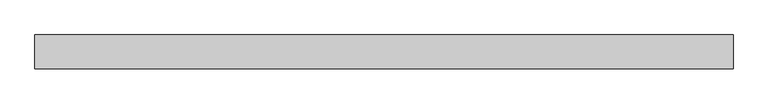
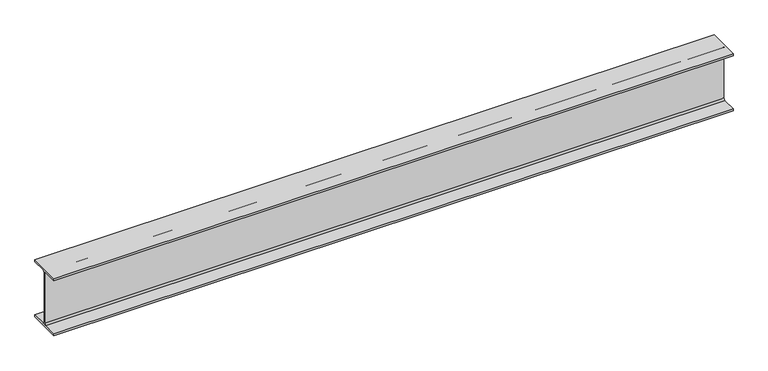
"""IFC4 building model written with IfcOpenShell, lengths in millimetres: beam geometry, Old_Steel Beam_H-KSD3502 : H_SB_ASB_H-200×200x8x12."""

import ifcopenshell
import ifcopenshell.guid

model = None  # the IFC model being written
_history = None  # IfcOwnerHistory: only IFC2X3 demands one
_inside = {}  # id of a spatial element -> (the spatial element, [elements in it])
_under = {}  # id of a project, library or spatial element -> (it, [spatial elements below it])
_declared = {}  # id of a project -> (the project, [libraries it declares])
_typed = {}  # id of a type object -> (the type object, [elements of that type])
_made_of = {}  # id of a material, layer set ... -> (it, [elements and type objects made of it])


def new_model(schema):
    """Start an empty IFC model of exactly this schema.

    Asked for "IFC4X3", IfcOpenShell would pick the latest addendum, in which some entities
    have other attributes; the version numbers below select the first issue.
    IFC2X3 requires an IfcOwnerHistory on every rooted entity: one is made here for all.
    """
    global model, _history
    if schema == "IFC4X3":
        model = ifcopenshell.file(schema_version=(4, 3, 0, 0))
    else:
        model = ifcopenshell.file(schema=schema)
    _inside.clear()
    _under.clear()
    _declared.clear()
    _typed.clear()
    _made_of.clear()
    _history = None
    if model.schema == "IFC2X3":
        org = make("IfcOrganization", Name="unknown")
        user = make(
            "IfcPersonAndOrganization",
            ThePerson=make("IfcPerson", FamilyName="unknown"),
            TheOrganization=org,
        )
        app = make(
            "IfcApplication",
            ApplicationDeveloper=org,
            Version="unknown",
            ApplicationFullName="unknown",
            ApplicationIdentifier="unknown",
        )
        _history = make(
            "IfcOwnerHistory",
            OwningUser=user,
            OwningApplication=app,
            ChangeAction="ADDED",
            CreationDate=0,
        )
    return model


def make(cls, **values):
    """One entity of the class cls with the attributes given. An attribute that is None is left unset."""
    return model.create_entity(
        cls, **{name: value for name, value in values.items() if value is not None}
    )


def rooted(cls, **values):
    """An entity with a GlobalId (a new one), such as an element, a storey or a relation."""
    return make(cls, GlobalId=ifcopenshell.guid.new(), OwnerHistory=_history, **values)


def si_unit(unit_type, name, prefix=None):
    """IfcSIUnit, for example si_unit("LENGTHUNIT", "METRE", prefix="MILLI")."""
    return make("IfcSIUnit", UnitType=unit_type, Prefix=prefix, Name=name)


def assignment(units):
    """IfcUnitAssignment: the units of a project."""
    return None if units is None else make("IfcUnitAssignment", Units=units)


def point(xyz):
    """IfcCartesianPoint."""
    return None if xyz is None else make("IfcCartesianPoint", Coordinates=xyz)


def direction(xyz):
    """IfcDirection."""
    return None if xyz is None else make("IfcDirection", DirectionRatios=xyz)


def frame(location, z_axis=None, x_axis=None):
    """IfcAxis2Placement3D, a coordinate frame: its origin and axes. An axis left out is left unset."""
    return make(
        "IfcAxis2Placement3D",
        Location=point(location),
        Axis=direction(z_axis),
        RefDirection=direction(x_axis),
    )


def frame_2d(location, x_axis=None):
    """IfcAxis2Placement2D, a coordinate frame in the plane: its origin and x axis."""
    return make(
        "IfcAxis2Placement2D", Location=point(location), RefDirection=direction(x_axis)
    )


def origin():
    """The frame at (0, 0, 0) with its axes left unset."""
    return frame((0.0, 0.0, 0.0))


def place(relative_to, where):
    """IfcLocalPlacement: puts the frame where relative to a parent placement (None: the world)."""
    return make(
        "IfcLocalPlacement", PlacementRelTo=relative_to, RelativePlacement=where
    )


def context(
    kind, dimensions, precision=None, world=None, true_north=None, identifier=None
):
    """IfcGeometricRepresentationContext, for example the 3D "Model" context."""
    return make(
        "IfcGeometricRepresentationContext",
        ContextIdentifier=identifier,
        ContextType=kind,
        CoordinateSpaceDimension=dimensions,
        Precision=precision,
        WorldCoordinateSystem=world,
        TrueNorth=true_north,
    )


def project(units=None, contexts=None):
    """IfcProject with its units and contexts."""
    return rooted(
        "IfcProject",
        Name="project",
        RepresentationContexts=contexts,
        UnitsInContext=assignment(units),
    )


def spatial(cls, under=None, at=None, **own):
    """A site, building, storey or space (cls), placed at a placement, below another one or the project."""
    s = rooted(cls, ObjectPlacement=at, **own)
    if under is not None:
        _under.setdefault(under.id(), (under, []))[1].append(s)
    return s


def polyline(points):
    """IfcPolyline through the points."""
    return make("IfcPolyline", Points=[point(p) for p in points])


def circle_curve(where, radius):
    """IfcCircle in the frame where."""
    return make("IfcCircle", Position=where, Radius=radius)


def trimmed(basis, trim1, trim2, sense, master):
    """IfcTrimmedCurve: the piece of a basis curve between two trims."""
    return make(
        "IfcTrimmedCurve",
        BasisCurve=basis,
        Trim1=trim1,
        Trim2=trim2,
        SenseAgreement=sense,
        MasterRepresentation=master,
    )


def segment(curve, same_sense, transition):
    """IfcCompositeCurveSegment."""
    return make(
        "IfcCompositeCurveSegment",
        Transition=transition,
        SameSense=same_sense,
        ParentCurve=curve,
    )


def composite_curve(segments, self_intersect=None):
    """IfcCompositeCurve: segments joined end to end."""
    return make("IfcCompositeCurve", Segments=segments, SelfIntersect=self_intersect)


def outline(outer, holes=None, kind="AREA"):
    """IfcArbitraryClosedProfileDef: a profile drawn as a closed curve; with holes, ...WithVoids."""
    if holes is None:
        return make("IfcArbitraryClosedProfileDef", ProfileType=kind, OuterCurve=outer)
    return make(
        "IfcArbitraryProfileDefWithVoids",
        ProfileType=kind,
        OuterCurve=outer,
        InnerCurves=holes,
    )


def extrude(swept, where, along, depth):
    """IfcExtrudedAreaSolid: the profile swept, set in the frame where, extruded along a direction by depth."""
    return make(
        "IfcExtrudedAreaSolid",
        SweptArea=swept,
        Position=where,
        ExtrudedDirection=direction(along),
        Depth=depth,
    )


def shape(context_of_items, identifier, shape_type, items):
    """IfcShapeRepresentation: the items that make up one representation, for example the "Body"."""
    return make(
        "IfcShapeRepresentation",
        ContextOfItems=context_of_items,
        RepresentationIdentifier=identifier,
        RepresentationType=shape_type,
        Items=items,
    )


def source(mapping_origin, context_of_items, identifier, shape_type, items):
    """IfcRepresentationMap: a shape defined once, which mapped items show again and again."""
    return make(
        "IfcRepresentationMap",
        MappingOrigin=mapping_origin,
        MappedRepresentation=shape(context_of_items, identifier, shape_type, items),
    )


def transform(
    local_origin,
    x_axis=None,
    y_axis=None,
    z_axis=None,
    scale=None,
    scale2=None,
    scale3=None,
    uniform=True,
):
    """IfcCartesianTransformationOperator3D, or its non-uniform kind. x_axis, y_axis, z_axis: its Axis1, 2, 3."""
    if uniform:
        return make(
            "IfcCartesianTransformationOperator3D",
            Axis1=direction(x_axis),
            Axis2=direction(y_axis),
            LocalOrigin=point(local_origin),
            Scale=scale,
            Axis3=direction(z_axis),
        )
    return make(
        "IfcCartesianTransformationOperator3DnonUniform",
        Axis1=direction(x_axis),
        Axis2=direction(y_axis),
        LocalOrigin=point(local_origin),
        Scale=scale,
        Axis3=direction(z_axis),
        Scale2=scale2,
        Scale3=scale3,
    )


def mapped(mapping_source, mapping_target):
    """IfcMappedItem: shows the shape of a source again, moved by a transform."""
    return make(
        "IfcMappedItem", MappingSource=mapping_source, MappingTarget=mapping_target
    )


def made_of(thing, what):
    """Note that an element or type object is made of a material, layer set ...; save() writes the relation."""
    if what is not None:
        _made_of.setdefault(what.id(), (what, []))[1].append(thing)
    return thing


def element(
    cls,
    number,
    at=None,
    inside=None,
    cuts=None,
    type_object=None,
    material=None,
    context=None,
    identifier="Body",
    shape_type=None,
    held_by="IfcProductDefinitionShape",
    body=None,
    shapes=None,
    **own,
):
    """One element of the class cls, such as IfcWall. Its Tag is "e" and its number.

    at: its placement. inside: the storey or other place that contains it. cuts: it is an
    opening in that element (IfcRelVoidsElement). A single representation is given by context,
    identifier, shape_type and body (its items); several are given by shapes. held_by: the class
    of the entity that holds the representations. save() writes the other relations.
    """
    e = rooted(cls, Tag="e%d" % number, ObjectPlacement=at, **own)
    if body is not None:
        shapes = [shape(context, identifier, shape_type, body)]
    if shapes is not None:
        e.Representation = make(held_by, Representations=shapes)
    if inside is not None:
        _inside.setdefault(inside.id(), (inside, []))[1].append(e)
    if cuts is not None:
        rooted(
            "IfcRelVoidsElement", RelatingBuildingElement=cuts, RelatedOpeningElement=e
        )
    if type_object is not None:
        _typed.setdefault(type_object.id(), (type_object, []))[1].append(e)
    return made_of(e, material)


def aggregate(whole, parts):
    """IfcRelAggregates: a whole, such as a stair, and the parts it consists of."""
    return rooted("IfcRelAggregates", RelatingObject=whole, RelatedObjects=parts)


def save(model, path):
    """Write the relations noted so far, then the file.

    IfcRelAggregates (storeys below a building ...), IfcRelContainedInSpatialStructure (elements
    in a storey), IfcRelDefinesByType, IfcRelAssociatesMaterial and IfcRelDeclares: one each for
    every whole, place, type object, material and project.
    """
    for whole, parts in _under.values():
        aggregate(whole, parts)
    for where, things in _inside.values():
        rooted(
            "IfcRelContainedInSpatialStructure",
            RelatedElements=things,
            RelatingStructure=where,
        )
    for kind, things in _typed.values():
        rooted("IfcRelDefinesByType", RelatedObjects=things, RelatingType=kind)
    for what, things in _made_of.values():
        rooted("IfcRelAssociatesMaterial", RelatedObjects=things, RelatingMaterial=what)
    for by, libraries in _declared.values():
        rooted("IfcRelDeclares", RelatingContext=by, RelatedDefinitions=libraries)
    model.write(path)


def beam_af1dc2e2(model_context):
    return source(origin(), model_context, "Body", "SweptSolid", [
        extrude(outline(composite_curve([segment(polyline([(-82.5, -141.5), (-11.9, -141.5)]), True, "CONTINUOUS"), segment(trimmed(circle_curve(frame_2d((-11.9, -132.6)), 8.9), [point((-11.9, -141.5))], [point((-3.0, -132.6))], True, "CARTESIAN"), True, "CONTINUOUS"), segment(polyline([(-3.0, -132.6), (-3.0, 132.6)]), True, "CONTINUOUS"), segment(trimmed(circle_curve(frame_2d((-11.9, 132.6)), 8.9), [point((-3.0, 132.6))], [point((-11.9, 141.5))], True, "CARTESIAN"), True, "CONTINUOUS"), segment(polyline([(-11.9, 141.5), (-82.5, 141.5), (-82.5, 151.7), (82.5, 151.7), (82.5, 141.5), (11.9, 141.5)]), True, "CONTINUOUS"), segment(trimmed(circle_curve(frame_2d((11.9, 132.6)), 8.9), [point((11.9, 141.5))], [point((3.0, 132.6))], True, "CARTESIAN"), True, "CONTINUOUS"), segment(polyline([(3.0, 132.6), (3.0, -132.6)]), True, "CONTINUOUS"), segment(trimmed(circle_curve(frame_2d((11.9, -132.6)), 8.9), [point((3.0, -132.6))], [point((11.9, -141.5))], True, "CARTESIAN"), True, "CONTINUOUS"), segment(polyline([(11.9, -141.5), (82.5, -141.5), (82.5, -151.7), (-82.5, -151.7), (-82.5, -141.5)]), True, "CONTINUOUS")], self_intersect=False)), frame((-1723.3906006, 0.0, 0.0), z_axis=(1.0, 0.0, 0.0), x_axis=(0.0, 1.0, 0.0)), (0.0, 0.0, 1.0), 3418.749313),
    ])


if __name__ == "__main__":
    model = new_model("IFC4")
    model_context = context("Model", 3, world=origin())
    ifc_project = project(units=[si_unit("LENGTHUNIT", "METRE", prefix="MILLI")], contexts=[model_context])
    site = spatial("IfcSite", under=ifc_project)
    building = spatial("IfcBuilding", under=site)
    placement = place(None, origin())
    beam_shape = beam_af1dc2e2(model_context)
    element("IfcBeam", 1, ObjectType="Old_Steel Beam_H-KSD3502 : H_SB_ASB_H-200×200x8x12", at=placement, inside=building, context=model_context, shape_type="MappedRepresentation", body=[
        mapped(beam_shape, transform((0.0, 0.0, 0.0), x_axis=(1.0, 0.0, 0.0), y_axis=(0.0, 1.0, 0.0), z_axis=(0.0, 0.0, 1.0))),
    ])
    save(model, "model.ifc")

# Revit data of these elements
# Type "Old_Steel Beam_H-KSD3502 : H_SB_ASB_H-200×200x8x12"
#   Width = 20.0 cm
#   Web Thickness = 0.8 cm
#   Web Fillet = 1.3 cm
#   Warping Constant = 141376.0 cm⁶
#   Torsional Moment of Inertia = 26.2485 cm⁴
#   Torsional Modulus = 1.0 cm³
#   Section Area = 63.53 cm²
#   Plastic Modulus weak axis = 244.0 cm³
#   Plastic Modulus strong axis = 525.0 cm³
#   Perimeter = 1.16 m²/m
#   Nominal Weight = 49.90 kgf/m
#   Moment of Inertia weak axis = 1600.00 cm⁴
#   Moment of Inertia strong axis = 4720.00 cm⁴
#   Height = 20.0 cm
#   Flange Thickness = 1.2 cm
#   Elastic Modulus weak axis = 160.0 cm³
#   Elastic Modulus strong axis = 472.0 cm³
#   Centroid Vertical = 10.0 cm
#   Centroid Horizontal = 10.0 cm
#   Length [instance default] = 1.5240 m
#   Structural Material [instance default] = Steel, 45-345
#   Assembly Code = ""
# Element 1 (IfcBeam, "Old_Steel Beam_H-KSD3502 : H_SB_ASB_H-200×200x8x12")
#   Structural Material = none
# Materials
#   "Steel, 45-345": class "Metal", colour RGB 189 187 185, transparency 0, Description = "Steel 345 MPa", Cost = 0
